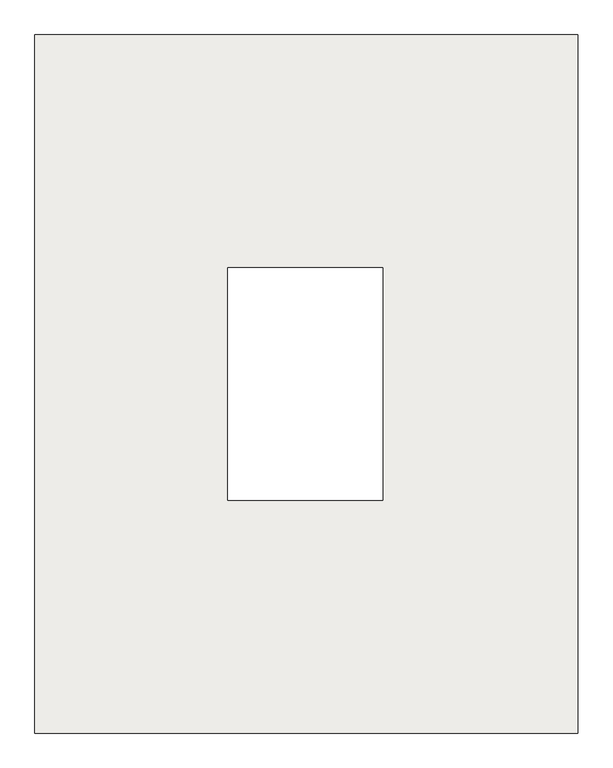
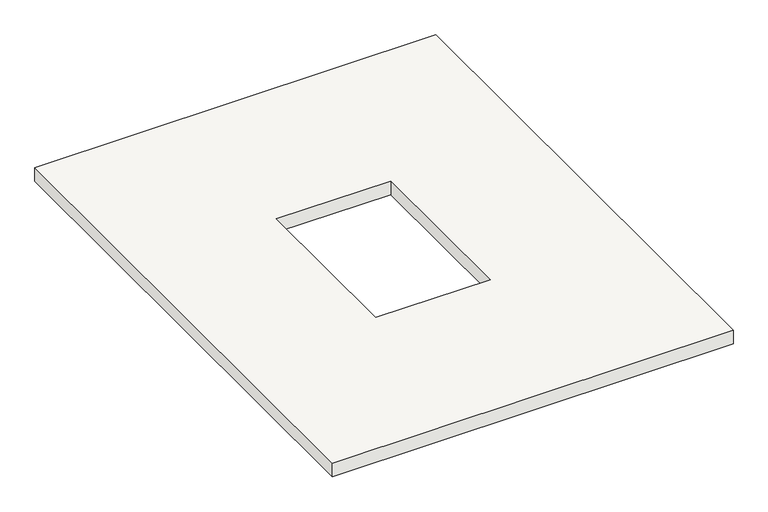
"""IFC4 building model written with IfcOpenShell, lengths in millimetres: slab geometry, Holzdecke : Holzdecke."""

import ifcopenshell
import ifcopenshell.guid

model = None  # the IFC model being written
_history = None  # IfcOwnerHistory: only IFC2X3 demands one
_inside = {}  # id of a spatial element -> (the spatial element, [elements in it])
_under = {}  # id of a project, library or spatial element -> (it, [spatial elements below it])
_declared = {}  # id of a project -> (the project, [libraries it declares])
_typed = {}  # id of a type object -> (the type object, [elements of that type])
_made_of = {}  # id of a material, layer set ... -> (it, [elements and type objects made of it])


def new_model(schema):
    """Start an empty IFC model of exactly this schema.

    Asked for "IFC4X3", IfcOpenShell would pick the latest addendum, in which some entities
    have other attributes; the version numbers below select the first issue.
    IFC2X3 requires an IfcOwnerHistory on every rooted entity: one is made here for all.
    """
    global model, _history
    if schema == "IFC4X3":
        model = ifcopenshell.file(schema_version=(4, 3, 0, 0))
    else:
        model = ifcopenshell.file(schema=schema)
    _inside.clear()
    _under.clear()
    _declared.clear()
    _typed.clear()
    _made_of.clear()
    _history = None
    if model.schema == "IFC2X3":
        org = make("IfcOrganization", Name="unknown")
        user = make(
            "IfcPersonAndOrganization",
            ThePerson=make("IfcPerson", FamilyName="unknown"),
            TheOrganization=org,
        )
        app = make(
            "IfcApplication",
            ApplicationDeveloper=org,
            Version="unknown",
            ApplicationFullName="unknown",
            ApplicationIdentifier="unknown",
        )
        _history = make(
            "IfcOwnerHistory",
            OwningUser=user,
            OwningApplication=app,
            ChangeAction="ADDED",
            CreationDate=0,
        )
    return model


def make(cls, **values):
    """One entity of the class cls with the attributes given. An attribute that is None is left unset."""
    return model.create_entity(
        cls, **{name: value for name, value in values.items() if value is not None}
    )


def rooted(cls, **values):
    """An entity with a GlobalId (a new one), such as an element, a storey or a relation."""
    return make(cls, GlobalId=ifcopenshell.guid.new(), OwnerHistory=_history, **values)


def si_unit(unit_type, name, prefix=None):
    """IfcSIUnit, for example si_unit("LENGTHUNIT", "METRE", prefix="MILLI")."""
    return make("IfcSIUnit", UnitType=unit_type, Prefix=prefix, Name=name)


def assignment(units):
    """IfcUnitAssignment: the units of a project."""
    return None if units is None else make("IfcUnitAssignment", Units=units)


def point(xyz):
    """IfcCartesianPoint."""
    return None if xyz is None else make("IfcCartesianPoint", Coordinates=xyz)


def direction(xyz):
    """IfcDirection."""
    return None if xyz is None else make("IfcDirection", DirectionRatios=xyz)


def frame(location, z_axis=None, x_axis=None):
    """IfcAxis2Placement3D, a coordinate frame: its origin and axes. An axis left out is left unset."""
    return make(
        "IfcAxis2Placement3D",
        Location=point(location),
        Axis=direction(z_axis),
        RefDirection=direction(x_axis),
    )


def origin():
    """The frame at (0, 0, 0) with its axes left unset."""
    return frame((0.0, 0.0, 0.0))


def place(relative_to, where):
    """IfcLocalPlacement: puts the frame where relative to a parent placement (None: the world)."""
    return make(
        "IfcLocalPlacement", PlacementRelTo=relative_to, RelativePlacement=where
    )


def context(
    kind, dimensions, precision=None, world=None, true_north=None, identifier=None
):
    """IfcGeometricRepresentationContext, for example the 3D "Model" context."""
    return make(
        "IfcGeometricRepresentationContext",
        ContextIdentifier=identifier,
        ContextType=kind,
        CoordinateSpaceDimension=dimensions,
        Precision=precision,
        WorldCoordinateSystem=world,
        TrueNorth=true_north,
    )


def project(units=None, contexts=None):
    """IfcProject with its units and contexts."""
    return rooted(
        "IfcProject",
        Name="project",
        RepresentationContexts=contexts,
        UnitsInContext=assignment(units),
    )


def spatial(cls, under=None, at=None, **own):
    """A site, building, storey or space (cls), placed at a placement, below another one or the project."""
    s = rooted(cls, ObjectPlacement=at, **own)
    if under is not None:
        _under.setdefault(under.id(), (under, []))[1].append(s)
    return s


def polyline(points):
    """IfcPolyline through the points."""
    return make("IfcPolyline", Points=[point(p) for p in points])


def outline(outer, holes=None, kind="AREA"):
    """IfcArbitraryClosedProfileDef: a profile drawn as a closed curve; with holes, ...WithVoids."""
    if holes is None:
        return make("IfcArbitraryClosedProfileDef", ProfileType=kind, OuterCurve=outer)
    return make(
        "IfcArbitraryProfileDefWithVoids",
        ProfileType=kind,
        OuterCurve=outer,
        InnerCurves=holes,
    )


def extrude(swept, where, along, depth):
    """IfcExtrudedAreaSolid: the profile swept, set in the frame where, extruded along a direction by depth."""
    return make(
        "IfcExtrudedAreaSolid",
        SweptArea=swept,
        Position=where,
        ExtrudedDirection=direction(along),
        Depth=depth,
    )


def shape(context_of_items, identifier, shape_type, items):
    """IfcShapeRepresentation: the items that make up one representation, for example the "Body"."""
    return make(
        "IfcShapeRepresentation",
        ContextOfItems=context_of_items,
        RepresentationIdentifier=identifier,
        RepresentationType=shape_type,
        Items=items,
    )


def source(mapping_origin, context_of_items, identifier, shape_type, items):
    """IfcRepresentationMap: a shape defined once, which mapped items show again and again."""
    return make(
        "IfcRepresentationMap",
        MappingOrigin=mapping_origin,
        MappedRepresentation=shape(context_of_items, identifier, shape_type, items),
    )


def transform(
    local_origin,
    x_axis=None,
    y_axis=None,
    z_axis=None,
    scale=None,
    scale2=None,
    scale3=None,
    uniform=True,
):
    """IfcCartesianTransformationOperator3D, or its non-uniform kind. x_axis, y_axis, z_axis: its Axis1, 2, 3."""
    if uniform:
        return make(
            "IfcCartesianTransformationOperator3D",
            Axis1=direction(x_axis),
            Axis2=direction(y_axis),
            LocalOrigin=point(local_origin),
            Scale=scale,
            Axis3=direction(z_axis),
        )
    return make(
        "IfcCartesianTransformationOperator3DnonUniform",
        Axis1=direction(x_axis),
        Axis2=direction(y_axis),
        LocalOrigin=point(local_origin),
        Scale=scale,
        Axis3=direction(z_axis),
        Scale2=scale2,
        Scale3=scale3,
    )


def mapped(mapping_source, mapping_target):
    """IfcMappedItem: shows the shape of a source again, moved by a transform."""
    return make(
        "IfcMappedItem", MappingSource=mapping_source, MappingTarget=mapping_target
    )


def made_of(thing, what):
    """Note that an element or type object is made of a material, layer set ...; save() writes the relation."""
    if what is not None:
        _made_of.setdefault(what.id(), (what, []))[1].append(thing)
    return thing


def element(
    cls,
    number,
    at=None,
    inside=None,
    cuts=None,
    type_object=None,
    material=None,
    context=None,
    identifier="Body",
    shape_type=None,
    held_by="IfcProductDefinitionShape",
    body=None,
    shapes=None,
    **own,
):
    """One element of the class cls, such as IfcWall. Its Tag is "e" and its number.

    at: its placement. inside: the storey or other place that contains it. cuts: it is an
    opening in that element (IfcRelVoidsElement). A single representation is given by context,
    identifier, shape_type and body (its items); several are given by shapes. held_by: the class
    of the entity that holds the representations. save() writes the other relations.
    """
    e = rooted(cls, Tag="e%d" % number, ObjectPlacement=at, **own)
    if body is not None:
        shapes = [shape(context, identifier, shape_type, body)]
    if shapes is not None:
        e.Representation = make(held_by, Representations=shapes)
    if inside is not None:
        _inside.setdefault(inside.id(), (inside, []))[1].append(e)
    if cuts is not None:
        rooted(
            "IfcRelVoidsElement", RelatingBuildingElement=cuts, RelatedOpeningElement=e
        )
    if type_object is not None:
        _typed.setdefault(type_object.id(), (type_object, []))[1].append(e)
    return made_of(e, material)


def aggregate(whole, parts):
    """IfcRelAggregates: a whole, such as a stair, and the parts it consists of."""
    return rooted("IfcRelAggregates", RelatingObject=whole, RelatedObjects=parts)


def save(model, path):
    """Write the relations noted so far, then the file.

    IfcRelAggregates (storeys below a building ...), IfcRelContainedInSpatialStructure (elements
    in a storey), IfcRelDefinesByType, IfcRelAssociatesMaterial and IfcRelDeclares: one each for
    every whole, place, type object, material and project.
    """
    for whole, parts in _under.values():
        aggregate(whole, parts)
    for where, things in _inside.values():
        rooted(
            "IfcRelContainedInSpatialStructure",
            RelatedElements=things,
            RelatingStructure=where,
        )
    for kind, things in _typed.values():
        rooted("IfcRelDefinesByType", RelatedObjects=things, RelatingType=kind)
    for what, things in _made_of.values():
        rooted("IfcRelAssociatesMaterial", RelatedObjects=things, RelatingMaterial=what)
    for by, libraries in _declared.values():
        rooted("IfcRelDeclares", RelatingContext=by, RelatedDefinitions=libraries)
    model.write(path)


def slab_87d51967(model_context):
    return source(origin(), model_context, "Body", "SweptSolid", [
        extrude(outline(polyline([(15500.0, 1547.1380981), (1500.0, 1547.1380981), (1500.0, 19550.0), (15500.0, 19550.0), (15500.0, 1547.1380981)]), holes=[polyline([(10475.0, 13550.0), (6475.0, 13550.0), (6475.0, 7550.0), (10475.0, 7550.0), (10475.0, 13550.0)])]), frame((0.0, 0.0, -500.0), z_axis=(0.0, 0.0, 1.0), x_axis=(1.0, 0.0, 0.0)), (0.0, 0.0, 1.0), 500.0),
    ])


if __name__ == "__main__":
    model = new_model("IFC4")
    model_context = context("Model", 3, world=origin())
    ifc_project = project(units=[si_unit("LENGTHUNIT", "METRE", prefix="MILLI")], contexts=[model_context])
    site = spatial("IfcSite", under=ifc_project)
    building = spatial("IfcBuilding", under=site)
    placement = place(None, origin())
    slab_shape = slab_87d51967(model_context)
    element("IfcSlab", 1, ObjectType="Holzdecke : Holzdecke", at=placement, inside=building, context=model_context, shape_type="MappedRepresentation", body=[
        mapped(slab_shape, transform((0.0, 0.0, 0.0), x_axis=(1.0, 0.0, 0.0), y_axis=(0.0, 1.0, 0.0), z_axis=(0.0, 0.0, 1.0))),
    ])
    save(model, "model.ifc")

# Revit data of these elements
# Type "Holzdecke : Holzdecke"
#   Abrechnungsart = "m²"
#   Allright_Bauteil_ID = "0110De 0783954323"
#   Bezeichnung = "Holzdecke"
#   Codetext = "D-HOLZBALKEN1\\"
#   Gewerk = "Zimmer- und Holzbauarbeiten"
#   Material = "Holz"
#   Objektname = "Brettstapeldecke"
#   NameOverride = "Holzdecke"
#   Reference = "Holzdecke"
#   Status = "NEW"
#   PitchAngle = 0.00°
#   ThermalTransmittance = 0.0000 BTU/(h·ft²·°F)
#   2D Interaktion = yes
#   Combustible = no
#   Compartmentation = no
#   IsExternal = no
#   LoadBearing = yes
# Element 1 (IfcSlab, "Holzdecke : Holzdecke")
#   Materials on its faces: "Default Floor"
# Materials
#   "Default Floor": class "Miscellaneous", colour RGB 128 128 128, transparency 0, Cost = 0
